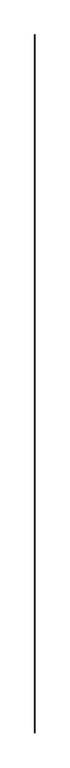
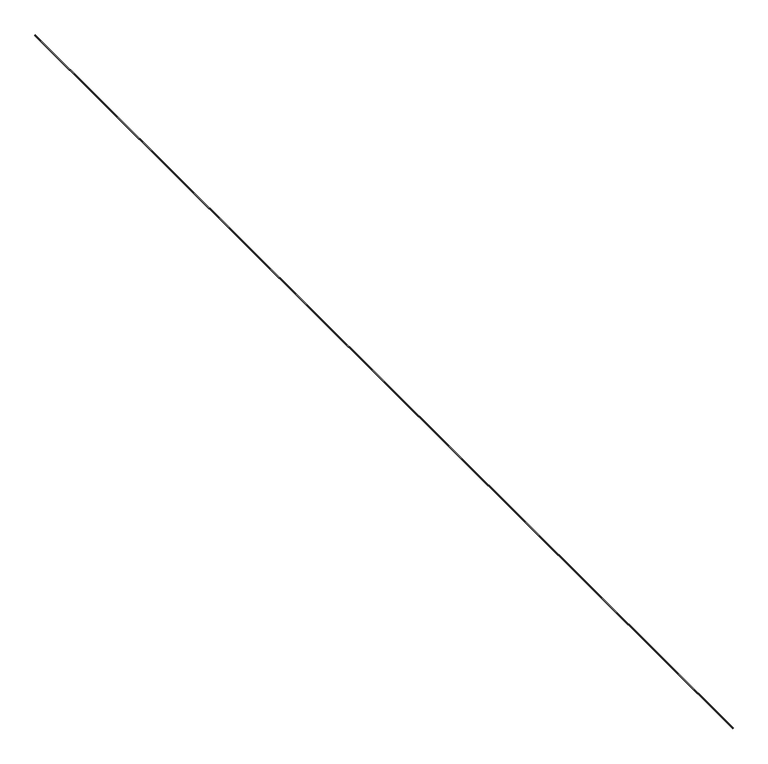
"""IFC4 building model written with IfcOpenShell, lengths in millimetres: proxy geometry, Inner panel:Inner panel:1:Inner panel:1 : Inner panel:Inner panel:300324:2:Inner panel:1:Inner panel:1 : Inner panel:Inner panel:300324:2 : Inner panel:Inner panel:1:Inner panel:1 : Inner panel:Inner panel:300324:300043:144 : Inner panel:Inner panel:1:Inner panel:1 : Inner panel:Inner panel:300324:2:Inner panel:1:Inner panel:1 : Inner panel:Inner panel:300324:2 : Inner panel:Inner panel:1:Inner panel:1 : Inner panel:Inner panel:300324:300043:308120."""

import ifcopenshell
import ifcopenshell.guid

model = None  # the IFC model being written
_history = None  # IfcOwnerHistory: only IFC2X3 demands one
_inside = {}  # id of a spatial element -> (the spatial element, [elements in it])
_under = {}  # id of a project, library or spatial element -> (it, [spatial elements below it])
_declared = {}  # id of a project -> (the project, [libraries it declares])
_typed = {}  # id of a type object -> (the type object, [elements of that type])
_made_of = {}  # id of a material, layer set ... -> (it, [elements and type objects made of it])


def new_model(schema):
    """Start an empty IFC model of exactly this schema.

    Asked for "IFC4X3", IfcOpenShell would pick the latest addendum, in which some entities
    have other attributes; the version numbers below select the first issue.
    IFC2X3 requires an IfcOwnerHistory on every rooted entity: one is made here for all.
    """
    global model, _history
    if schema == "IFC4X3":
        model = ifcopenshell.file(schema_version=(4, 3, 0, 0))
    else:
        model = ifcopenshell.file(schema=schema)
    _inside.clear()
    _under.clear()
    _declared.clear()
    _typed.clear()
    _made_of.clear()
    _history = None
    if model.schema == "IFC2X3":
        org = make("IfcOrganization", Name="unknown")
        user = make(
            "IfcPersonAndOrganization",
            ThePerson=make("IfcPerson", FamilyName="unknown"),
            TheOrganization=org,
        )
        app = make(
            "IfcApplication",
            ApplicationDeveloper=org,
            Version="unknown",
            ApplicationFullName="unknown",
            ApplicationIdentifier="unknown",
        )
        _history = make(
            "IfcOwnerHistory",
            OwningUser=user,
            OwningApplication=app,
            ChangeAction="ADDED",
            CreationDate=0,
        )
    return model


def make(cls, **values):
    """One entity of the class cls with the attributes given. An attribute that is None is left unset."""
    return model.create_entity(
        cls, **{name: value for name, value in values.items() if value is not None}
    )


def rooted(cls, **values):
    """An entity with a GlobalId (a new one), such as an element, a storey or a relation."""
    return make(cls, GlobalId=ifcopenshell.guid.new(), OwnerHistory=_history, **values)


def si_unit(unit_type, name, prefix=None):
    """IfcSIUnit, for example si_unit("LENGTHUNIT", "METRE", prefix="MILLI")."""
    return make("IfcSIUnit", UnitType=unit_type, Prefix=prefix, Name=name)


def assignment(units):
    """IfcUnitAssignment: the units of a project."""
    return None if units is None else make("IfcUnitAssignment", Units=units)


def point(xyz):
    """IfcCartesianPoint."""
    return None if xyz is None else make("IfcCartesianPoint", Coordinates=xyz)


def direction(xyz):
    """IfcDirection."""
    return None if xyz is None else make("IfcDirection", DirectionRatios=xyz)


def frame(location, z_axis=None, x_axis=None):
    """IfcAxis2Placement3D, a coordinate frame: its origin and axes. An axis left out is left unset."""
    return make(
        "IfcAxis2Placement3D",
        Location=point(location),
        Axis=direction(z_axis),
        RefDirection=direction(x_axis),
    )


def origin():
    """The frame at (0, 0, 0) with its axes left unset."""
    return frame((0.0, 0.0, 0.0))


def place(relative_to, where):
    """IfcLocalPlacement: puts the frame where relative to a parent placement (None: the world)."""
    return make(
        "IfcLocalPlacement", PlacementRelTo=relative_to, RelativePlacement=where
    )


def context(
    kind, dimensions, precision=None, world=None, true_north=None, identifier=None
):
    """IfcGeometricRepresentationContext, for example the 3D "Model" context."""
    return make(
        "IfcGeometricRepresentationContext",
        ContextIdentifier=identifier,
        ContextType=kind,
        CoordinateSpaceDimension=dimensions,
        Precision=precision,
        WorldCoordinateSystem=world,
        TrueNorth=true_north,
    )


def project(units=None, contexts=None):
    """IfcProject with its units and contexts."""
    return rooted(
        "IfcProject",
        Name="project",
        RepresentationContexts=contexts,
        UnitsInContext=assignment(units),
    )


def spatial(cls, under=None, at=None, **own):
    """A site, building, storey or space (cls), placed at a placement, below another one or the project."""
    s = rooted(cls, ObjectPlacement=at, **own)
    if under is not None:
        _under.setdefault(under.id(), (under, []))[1].append(s)
    return s


def polyline(points):
    """IfcPolyline through the points."""
    return make("IfcPolyline", Points=[point(p) for p in points])


def outline(outer, holes=None, kind="AREA"):
    """IfcArbitraryClosedProfileDef: a profile drawn as a closed curve; with holes, ...WithVoids."""
    if holes is None:
        return make("IfcArbitraryClosedProfileDef", ProfileType=kind, OuterCurve=outer)
    return make(
        "IfcArbitraryProfileDefWithVoids",
        ProfileType=kind,
        OuterCurve=outer,
        InnerCurves=holes,
    )


def extrude(swept, where, along, depth):
    """IfcExtrudedAreaSolid: the profile swept, set in the frame where, extruded along a direction by depth."""
    return make(
        "IfcExtrudedAreaSolid",
        SweptArea=swept,
        Position=where,
        ExtrudedDirection=direction(along),
        Depth=depth,
    )


def shape(context_of_items, identifier, shape_type, items):
    """IfcShapeRepresentation: the items that make up one representation, for example the "Body"."""
    return make(
        "IfcShapeRepresentation",
        ContextOfItems=context_of_items,
        RepresentationIdentifier=identifier,
        RepresentationType=shape_type,
        Items=items,
    )


def source(mapping_origin, context_of_items, identifier, shape_type, items):
    """IfcRepresentationMap: a shape defined once, which mapped items show again and again."""
    return make(
        "IfcRepresentationMap",
        MappingOrigin=mapping_origin,
        MappedRepresentation=shape(context_of_items, identifier, shape_type, items),
    )


def transform(
    local_origin,
    x_axis=None,
    y_axis=None,
    z_axis=None,
    scale=None,
    scale2=None,
    scale3=None,
    uniform=True,
):
    """IfcCartesianTransformationOperator3D, or its non-uniform kind. x_axis, y_axis, z_axis: its Axis1, 2, 3."""
    if uniform:
        return make(
            "IfcCartesianTransformationOperator3D",
            Axis1=direction(x_axis),
            Axis2=direction(y_axis),
            LocalOrigin=point(local_origin),
            Scale=scale,
            Axis3=direction(z_axis),
        )
    return make(
        "IfcCartesianTransformationOperator3DnonUniform",
        Axis1=direction(x_axis),
        Axis2=direction(y_axis),
        LocalOrigin=point(local_origin),
        Scale=scale,
        Axis3=direction(z_axis),
        Scale2=scale2,
        Scale3=scale3,
    )


def mapped(mapping_source, mapping_target):
    """IfcMappedItem: shows the shape of a source again, moved by a transform."""
    return make(
        "IfcMappedItem", MappingSource=mapping_source, MappingTarget=mapping_target
    )


def made_of(thing, what):
    """Note that an element or type object is made of a material, layer set ...; save() writes the relation."""
    if what is not None:
        _made_of.setdefault(what.id(), (what, []))[1].append(thing)
    return thing


def element(
    cls,
    number,
    at=None,
    inside=None,
    cuts=None,
    type_object=None,
    material=None,
    context=None,
    identifier="Body",
    shape_type=None,
    held_by="IfcProductDefinitionShape",
    body=None,
    shapes=None,
    **own,
):
    """One element of the class cls, such as IfcWall. Its Tag is "e" and its number.

    at: its placement. inside: the storey or other place that contains it. cuts: it is an
    opening in that element (IfcRelVoidsElement). A single representation is given by context,
    identifier, shape_type and body (its items); several are given by shapes. held_by: the class
    of the entity that holds the representations. save() writes the other relations.
    """
    e = rooted(cls, Tag="e%d" % number, ObjectPlacement=at, **own)
    if body is not None:
        shapes = [shape(context, identifier, shape_type, body)]
    if shapes is not None:
        e.Representation = make(held_by, Representations=shapes)
    if inside is not None:
        _inside.setdefault(inside.id(), (inside, []))[1].append(e)
    if cuts is not None:
        rooted(
            "IfcRelVoidsElement", RelatingBuildingElement=cuts, RelatedOpeningElement=e
        )
    if type_object is not None:
        _typed.setdefault(type_object.id(), (type_object, []))[1].append(e)
    return made_of(e, material)


def aggregate(whole, parts):
    """IfcRelAggregates: a whole, such as a stair, and the parts it consists of."""
    return rooted("IfcRelAggregates", RelatingObject=whole, RelatedObjects=parts)


def save(model, path):
    """Write the relations noted so far, then the file.

    IfcRelAggregates (storeys below a building ...), IfcRelContainedInSpatialStructure (elements
    in a storey), IfcRelDefinesByType, IfcRelAssociatesMaterial and IfcRelDeclares: one each for
    every whole, place, type object, material and project.
    """
    for whole, parts in _under.values():
        aggregate(whole, parts)
    for where, things in _inside.values():
        rooted(
            "IfcRelContainedInSpatialStructure",
            RelatedElements=things,
            RelatingStructure=where,
        )
    for kind, things in _typed.values():
        rooted("IfcRelDefinesByType", RelatedObjects=things, RelatingType=kind)
    for what, things in _made_of.values():
        rooted("IfcRelAssociatesMaterial", RelatedObjects=things, RelatingMaterial=what)
    for by, libraries in _declared.values():
        rooted("IfcRelDeclares", RelatingContext=by, RelatedDefinitions=libraries)
    model.write(path)


def generic_models_440c6734(model_context):
    return source(origin(), model_context, "Body", "SweptSolid", [
        extrude(outline(polyline([(3907.7317159, 560268.8558776), (3909.3178397, 560306.9228477), (3947.3848098, 560305.3367239), (3945.798686, 560267.2697538), (3907.7317159, 560268.8558776)]), holes=[polyline([(3910.2100343, 560271.1359305), (3943.5186331, 560269.7480722), (3944.9064914, 560303.056671), (3911.5978926, 560304.4445293), (3910.2100343, 560271.1359305)])]), frame((0.0, -579346.5018007, 0.0), z_axis=(0.0, 1.0, 0.0), x_axis=(0.0, 0.0, 1.0)), (0.0, 0.0, 1.0), 88442.8),
    ])


if __name__ == "__main__":
    model = new_model("IFC4")
    model_context = context("Model", 3, world=origin())
    ifc_project = project(units=[si_unit("LENGTHUNIT", "METRE", prefix="MILLI")], contexts=[model_context])
    site = spatial("IfcSite", under=ifc_project)
    building = spatial("IfcBuilding", under=site)
    placement = place(None, origin())
    generic_models_shape = generic_models_440c6734(model_context)
    element("IfcBuildingElementProxy", 1, Name="Inner panel:Inner panel:1:Inner panel:1 : Inner panel:Inner panel:300324:2:Inner panel:1:Inner panel:1 : Inner panel:Inner panel:300324:2 : Inner panel:Inner panel:1:Inner panel:1 : Inner panel:Inner panel:300324:300043:144 : Inner panel:Inner panel:1:Inner panel:1 : Inner panel:Inner panel:300324:2:Inner panel:1:Inner panel:1 : Inner panel:Inner panel:300324:2 : Inner panel:Inner panel:1:Inner panel:1 : Inner panel:Inner panel:300324:300043:308120", ObjectType="Inner panel:Inner panel:1:Inner panel:1 : Inner panel:Inner panel:300324:2:Inner panel:1:Inner panel:1 : Inner panel:Inner panel:300324:2 : Inner panel:Inner panel:1:Inner panel:1 : Inner panel:Inner panel:300324:300043:144 : Inner panel:Inner panel:1:Inner panel:1 : Inner panel:Inner panel:300324:2:Inner panel:1:Inner panel:1 : Inner panel:Inner panel:300324:2 : Inner panel:Inner panel:1:Inner panel:1 : Inner panel:Inner panel:300324:300043:308120", at=placement, inside=building, context=model_context, shape_type="MappedRepresentation", body=[
        mapped(generic_models_shape, transform((0.0, 0.0, 0.0), x_axis=(1.0, 0.0, 0.0), y_axis=(0.0, 1.0, 0.0), z_axis=(0.0, 0.0, 1.0))),
    ])
    save(model, "model.ifc")

# Revit data of these elements
# Type "Inner panel:Inner panel:1:Inner panel:1 : Inner panel:Inner panel:300324:2:Inner panel:1:Inner panel:1 : Inner panel:Inner panel:300324:2 : Inner panel:Inner panel:1:Inner panel:1 : Inner panel:Inner panel:300324:300043:144 : Inner panel:Inner panel:1:Inner panel:1 : Inner panel:Inner panel:300324:2:Inner panel:1:Inner panel:1 : Inner panel:Inner panel:300324:2 : Inner panel:Inner panel:1:Inner panel:1 : Inner panel:Inner panel:300324:300043:308120"
#   NameOverride = "Inner panel:Inner panel:1:Inner panel:1 : Inner panel:Inner panel:300324:2:Inner panel:1:Inner panel:1 : Inner panel:Inner panel:300324:2 : Inner panel:Inner panel:1:Inner panel:1 : Inner panel:Inner panel:300324:300043:308120"
#   ObjectTypeOverride = "Inner panel:1:Inner panel:1 : Inner panel:Inner panel:300324:2 : Inner panel:Inner panel:1:Inner panel:1 : Inner panel:Inner panel:300324:300043"
#   Reference = "Inner panel"
#   Tag = "308120"
# Element 1 (IfcBuildingElementProxy, "Inner panel:Inner panel:1:Inner panel:1 : Inner panel:Inner panel:300324:2:Inner panel:1:Inner panel:1 : Inner panel:Inner panel:300324:2 : Inner panel:Inner panel:1:Inner panel:1 : Inner panel:Inner panel:300324:300043:144 : Inner panel:Inner panel:1:Inner panel:1 : Inner panel:Inner panel:300324:2:Inner panel:1:Inner panel:1 : Inner panel:Inner panel:300324:2 : Inner panel:Inner panel:1:Inner panel:1 : Inner panel:Inner panel:300324:300043:308120")
#   Materials on its faces: "1 1/2\" X 1 1/2\" x 1/8\" ALUM. TUBE (6061-T6) - (2) #16 WOOD SCREWS WITH 2.5\" EMBED AT EACH GLULAM - (1) SCREW AT ENDS"
# Materials
#   "1 1/2\" X 1 1/2\" x 1/8\" ALUM. TUBE (6061-T6) - (2) #16 WOOD SCREWS WITH 2.5\" EMBED AT EACH GLULAM - (1) SCREW AT ENDS": class "Unassigned", colour RGB 202 201 200, transparency 0, Cost = 0
